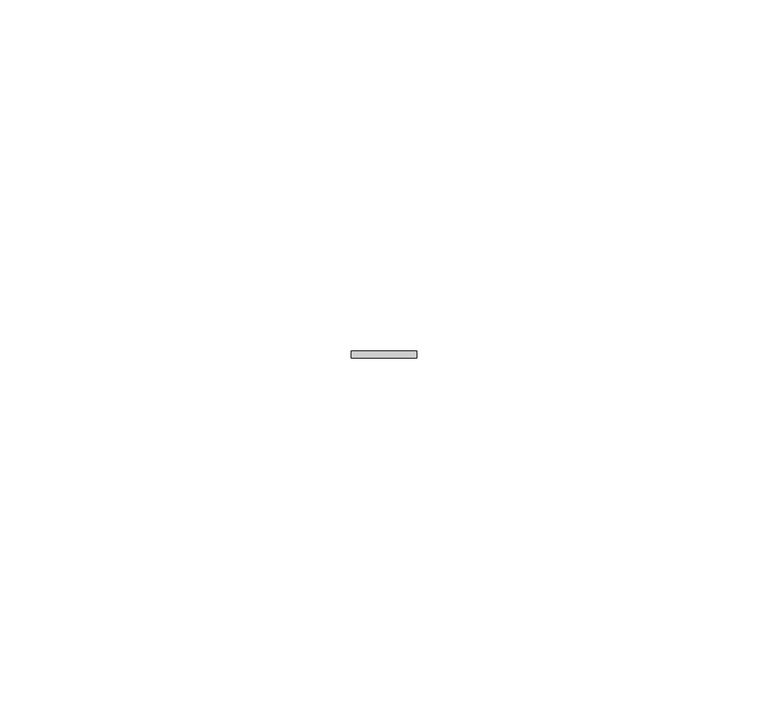
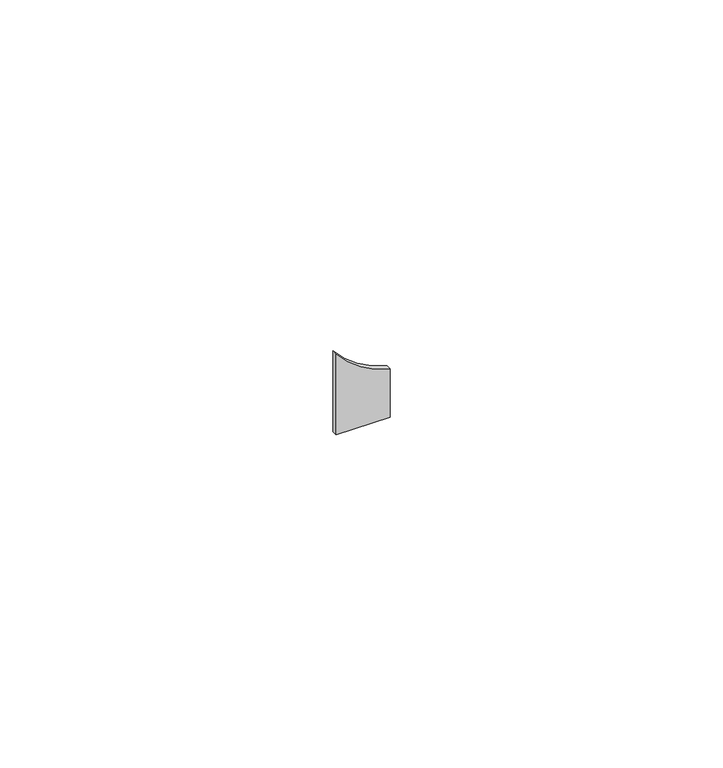
"""IFC4 building model written with IfcOpenShell, lengths in millimetres: proxy geometry, Joint046 6348 : Joint046 6348."""

from ifc_helpers import new_model, si_unit, point, frame, frame_2d, origin, place, context, project, spatial, polyline, circle_curve, trimmed, segment, composite_curve, outline, extrude, source, transform, mapped, element, save


def generic_models_c6a20d00(model_context):
    return source(origin(), model_context, "Body", "SweptSolid", [
        extrude(outline(composite_curve([segment(polyline([(40191.0775869, 10146.3892018), (40176.3050233, 10146.3892018), (40176.3050211, 10155.7382812), (40185.1257077, 10155.7382812)]), True, "CONTINUOUS"), segment(trimmed(circle_curve(frame_2d((40201.8444315, 10159.8127732)), 17.2080565), [point((40185.1257077, 10155.7382812))], [point((40191.0775869, 10146.3892018))], True, "CARTESIAN"), True, "CONTINUOUS")], self_intersect=False)), frame((0.0, 4216.3610002, 0.0), z_axis=(0.0, 1.0, 0.0), x_axis=(0.0, 0.0, 1.0)), (0.0, 0.0, 1.0), 1.0),
    ])


if __name__ == "__main__":
    model = new_model("IFC4")
    model_context = context("Model", 3, world=origin())
    ifc_project = project(units=[si_unit("LENGTHUNIT", "METRE", prefix="MILLI")], contexts=[model_context])
    site = spatial("IfcSite", under=ifc_project)
    building = spatial("IfcBuilding", under=site)
    placement = place(None, origin())
    generic_models_shape = generic_models_c6a20d00(model_context)
    element("IfcBuildingElementProxy", 1, Name="Joint046 6348 : Joint046 6348", ObjectType="Joint046 6348 : Joint046 6348", at=placement, inside=building, context=model_context, shape_type="MappedRepresentation", body=[
        mapped(generic_models_shape, transform((0.0, 0.0, 0.0), x_axis=(1.0, 0.0, 0.0), y_axis=(0.0, 1.0, 0.0), z_axis=(0.0, 0.0, 1.0))),
    ])
    save(model, "model.ifc")

# Revit data of these elements
# Type "Joint046 6348 : Joint046 6348"
#   NameOverride = "Joint046"
# Element 1 (IfcBuildingElementProxy, "Joint046 6348 : Joint046 6348")
#   Materials on its faces: "SEALANT"
# Materials
#   "SEALANT": class "Unassigned", colour RGB 142 225 148, transparency 0
